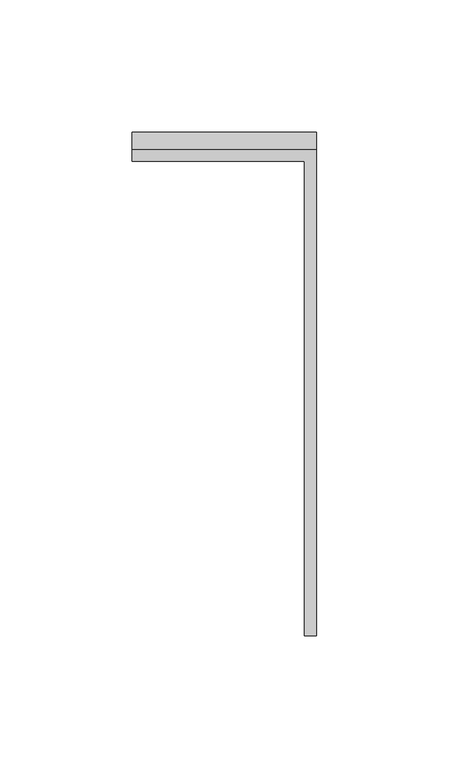
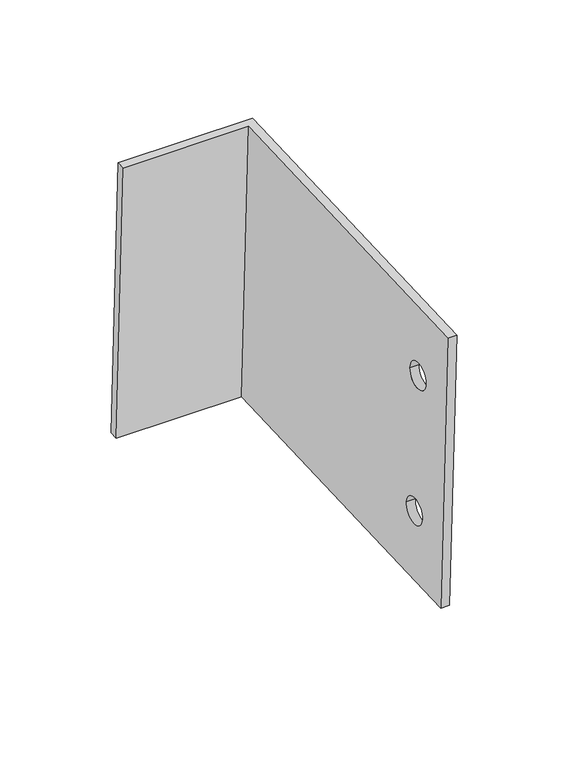
"""IFC4 building model written with IfcOpenShell, lengths in millimetres: proxy geometry, Generic Models 7:Generic Models 1:8:Generic Models 1:8 : Generic Models 7:Generic Models 1:337419:28 : Generic Models 7:Generic Models 1:8:Generic Models 1:8 : Generic Models 7:Generic Models 1:337419:315935."""

from ifc_helpers import new_model, si_unit, frame, origin, place, context, project, spatial, polyline, circle_curve, source, transform, mapped, element, save
from ifc_brep_helpers import plane_surface, revolved_surface, advanced_brep


def generic_models_fb0905f0(model_context):
    return source(origin(), model_context, "Body", "AdvancedBrep", [
        advanced_brep(
        [(593665.2601618, -564939.7244578, 8729.2523376), (593665.2601618, -564946.0689528, 8881.5202179), (593665.2601618, -564766.6387032, 8888.9964783), (593665.2601618, -564760.2942082, 8736.728598), (593665.2601618, -564911.961099, 8844.5106637), (593665.2601618, -564926.248599, 8844.5106637), (593665.2601618, -564908.8136132, 8768.9710043), (593665.2601618, -564923.0515898, 8767.7824427), (593669.8242243, -564939.7244578, 8729.2523376), (593669.8242243, -564946.0689528, 8881.5202179), (593669.8242243, -564926.248599, 8844.5106637), (593669.8242243, -564911.961099, 8844.5106637), (593669.8242243, -564923.0515898, 8767.7824427), (593669.8242243, -564908.8136132, 8768.9710043), (593599.9742243, -564755.7341024, 8736.9186024), (593599.9742243, -564762.0785974, 8889.1864827), (593669.8242243, -564762.0785974, 8889.1864827), (593669.8242243, -564755.7341024, 8736.9186024), (593599.9742243, -564766.6387032, 8888.9964783), (593599.9742243, -564760.2942082, 8736.728598)],
        [
            (0, 1),
            (1, 2),
            (2, 3),
            (3, 0),
            (4, 5, circle_curve(frame((593665.2601618, -564919.104849, 8844.5106637), z_axis=(1.0, 0.0, 0.0), x_axis=(0.0, -1.0, 0.0)), 7.14375)),
            (5, 4, circle_curve(frame((593665.2601618, -564919.104849, 8844.5106637), z_axis=(1.0, 0.0, 0.0), x_axis=(0.0, -1.0, 0.0)), 7.14375)),
            (6, 7, circle_curve(frame((593665.2601618, -564915.9326015, 8768.3767235), z_axis=(1.0, 0.0, 0.0), x_axis=(0.0, -0.9965337954939333, -0.08318890814559193)), 7.14375)),
            (7, 6, circle_curve(frame((593665.2601618, -564915.9326015, 8768.3767235), z_axis=(1.0, 0.0, 0.0), x_axis=(0.0, -0.9965337954939333, -0.08318890814559193)), 7.14375)),
            (0, 8),
            (8, 9),
            (9, 1),
            (5, 10),
            (10, 11, circle_curve(frame((593669.8242243, -564919.104849, 8844.5106637), z_axis=(1.0, 0.0, 0.0), x_axis=(0.0, -1.0, 0.0)), 7.14375)),
            (11, 4),
            (11, 10, circle_curve(frame((593669.8242243, -564919.104849, 8844.5106637), z_axis=(1.0, 0.0, 0.0), x_axis=(0.0, -1.0, 0.0)), 7.14375)),
            (7, 12),
            (12, 13, circle_curve(frame((593669.8242243, -564915.9326015, 8768.3767235), z_axis=(1.0, 0.0, 0.0), x_axis=(0.0, -0.9965337954939333, -0.08318890814559193)), 7.14375)),
            (13, 6),
            (13, 12, circle_curve(frame((593669.8242243, -564915.9326015, 8768.3767235), z_axis=(1.0, 0.0, 0.0), x_axis=(0.0, -0.9965337954939333, -0.08318890814559193)), 7.14375)),
            (14, 15),
            (15, 16),
            (16, 17),
            (17, 14),
            (18, 19),
            (19, 3),
            (2, 18),
            (14, 19),
            (18, 15),
            (17, 8),
            (16, 9),
        ],
        [
            plane_surface(frame((593665.2601618, -564986.8156465, 8727.2902047), z_axis=(-1.0000000000000002, 0.0, 0.0), x_axis=(0.0, -0.999133073092352, -0.04163054471218133))),
            plane_surface(frame((593669.8242243, -564946.0689528, 8881.5202179), z_axis=(0.0, -0.9991330730924919, -0.04163054470882304), x_axis=(-1.0, 0.0, 0.0))),
            revolved_surface(polyline([(593665.2601618, -564926.248599, 8844.5106637), (593669.8242243, -564926.248599, 8844.5106637)]), (588788.4601618, -564919.104849, 8844.5106637), (-1.0, 0.0, 0.0)),
            revolved_surface(polyline([(593665.2601618, -564923.0515898016, 8767.782442737434), (593669.8242243, -564923.0515898016, 8767.782442737434)]), (588788.4601618, -564915.9326015, 8768.3767235), (-1.0000000000000002, 0.0, 0.0)),
            plane_surface(frame((593443.1062381, -564755.7341024, 8736.9186024), z_axis=(-4.445379624845071e-12, 0.9991330730923519, 0.0416305447121838), x_axis=(-1.0, -4.4421706340813435e-12, 0.0))),
            plane_surface(frame((593443.1062381, -564760.2942082, 8736.728598), z_axis=(4.445379624845071e-12, -0.9991330730923519, -0.0416305447121838), x_axis=(1.0, 4.4421706340813435e-12, 0.0))),
            plane_surface(frame((593599.9742243, -564766.6387032, 8888.9964783), z_axis=(-1.0, 0.0, 3.634824945374381e-12), x_axis=(0.0, 0.9991330730923585, 0.04163054471202344))),
            plane_surface(frame((593599.9742243, -564760.2942082, 8736.728598), z_axis=(0.0, 0.04163054471226028, -0.9991330730923487), x_axis=(0.0, 0.9991330730923487, 0.04163054471226028))),
            plane_surface(frame((593669.8242243, -564760.2942082, 8736.728598), z_axis=(1.0, 0.0, 0.0), x_axis=(0.0, 0.9991330730923487, 0.04163054471226028))),
            plane_surface(frame((593669.8242243, -564766.6387032, 8888.9964783), z_axis=(0.0, -0.04163054471226028, 0.9991330730923487), x_axis=(0.0, 0.9991330730923487, 0.04163054471226028))),
        ],
        [
            (0, [[1, 2, 3, 4], [5, 6], [7, 8]]),
            (1, [[-1, 9, 10, 11]]),
            (2, [[-6, 12, 13, 14]]),
            (2, [[-5, -14, 15, -12]]),
            (3, [[-8, 16, 17, 18]]),
            (3, [[-7, -18, 19, -16]]),
            (4, [[20, 21, 22, 23]]),
            (5, [[24, 25, -3, 26]]),
            (6, [[-20, 27, -24, 28]]),
            (7, [[-23, 29, -9, -4, -25, -27]]),
            (8, [[-29, -22, 30, -10], [-13, -15], [-17, -19]]),
            (9, [[-30, -21, -28, -26, -2, -11]]),
        ],
    ),
    ])


if __name__ == "__main__":
    model = new_model("IFC4")
    model_context = context("Model", 3, world=origin())
    ifc_project = project(units=[si_unit("LENGTHUNIT", "METRE", prefix="MILLI")], contexts=[model_context])
    site = spatial("IfcSite", under=ifc_project)
    building = spatial("IfcBuilding", under=site)
    placement = place(None, origin())
    generic_models_shape = generic_models_fb0905f0(model_context)
    element("IfcBuildingElementProxy", 1, Name="Generic Models 7:Generic Models 1:8:Generic Models 1:8 : Generic Models 7:Generic Models 1:337419:28 : Generic Models 7:Generic Models 1:8:Generic Models 1:8 : Generic Models 7:Generic Models 1:337419:315935", ObjectType="Generic Models 7:Generic Models 1:8:Generic Models 1:8 : Generic Models 7:Generic Models 1:337419:28 : Generic Models 7:Generic Models 1:8:Generic Models 1:8 : Generic Models 7:Generic Models 1:337419:315935", at=placement, inside=building, context=model_context, shape_type="MappedRepresentation", body=[
        mapped(generic_models_shape, transform((0.0, 0.0, 0.0), x_axis=(1.0, 0.0, 0.0), y_axis=(0.0, 1.0, 0.0), z_axis=(0.0, 0.0, 1.0))),
    ])
    save(model, "model.ifc")

# Revit data of these elements
# Type "Generic Models 7:Generic Models 1:8:Generic Models 1:8 : Generic Models 7:Generic Models 1:337419:28 : Generic Models 7:Generic Models 1:8:Generic Models 1:8 : Generic Models 7:Generic Models 1:337419:315935"
#   NameOverride = "Generic Models 7:Generic Models 1:8:Generic Models 1:8 : Generic Models 7:Generic Models 1:337419:315935"
#   ObjectTypeOverride = "Generic Models 1:8 : Generic Models 7:Generic Models 1:337419"
#   Reference = "Generic Models 1"
#   Tag = "315935"
# Element 1 (IfcBuildingElementProxy, "Generic Models 7:Generic Models 1:8:Generic Models 1:8 : Generic Models 7:Generic Models 1:337419:28 : Generic Models 7:Generic Models 1:8:Generic Models 1:8 : Generic Models 7:Generic Models 1:337419:315935")
#   Materials on its faces: "0.179\" THICK BENT STEEL CLIPS"
# Materials
#   "0.179\" THICK BENT STEEL CLIPS": class "Metal", colour RGB 189 187 185, transparency 0, Description = "Structural steel 50ksi", Cost = 0
